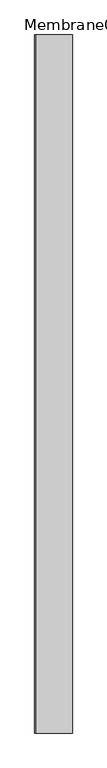
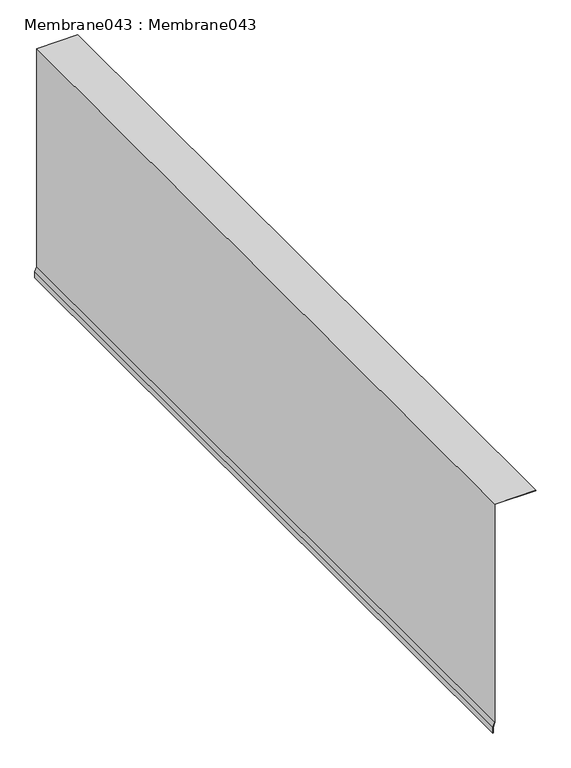
"""IFC4 building model written with IfcOpenShell, lengths in millimetres: proxy geometry, Membrane043 : Membrane043."""

from ifc_helpers import new_model, si_unit, frame, origin, place, context, project, spatial, polyline, outline, extrude, source, transform, mapped, element, save


def membrane043_membrane043_b5c9dd8e(model_context):
    return source(origin(), model_context, "Body", "SweptSolid", [
        extrude(outline(polyline([(40160.8681333, -9788.4545063), (40160.8681333, -9892.1962891), (39579.4993977, -9892.1962891), (39568.2741325, -9896.2819515), (39552.6918208, -9896.2819515), (39552.6918208, -9895.2819515), (39568.0978055, -9895.2819515), (39579.3230707, -9891.1962891), (40159.8681333, -9891.1962891), (40159.8681333, -9788.4545063), (40160.8681333, -9788.4545063)])), frame((0.0, 7982.1531721, 0.0), z_axis=(0.0, 1.0, 0.0), x_axis=(0.0, 0.0, 1.0)), (0.0, 0.0, 1.0), 2000.0),
    ])


if __name__ == "__main__":
    model = new_model("IFC4")
    model_context = context("Model", 3, world=origin())
    ifc_project = project(units=[si_unit("LENGTHUNIT", "METRE", prefix="MILLI")], contexts=[model_context])
    site = spatial("IfcSite", under=ifc_project)
    building = spatial("IfcBuilding", under=site)
    placement = place(None, origin())
    membrane043_membrane043_shape = membrane043_membrane043_b5c9dd8e(model_context)
    element("IfcBuildingElementProxy", 1, Name="Membrane043 : Membrane043", ObjectType="Membrane043 : Membrane043", at=placement, inside=building, context=model_context, shape_type="MappedRepresentation", body=[
        mapped(membrane043_membrane043_shape, transform((0.0, 0.0, 0.0), x_axis=(1.0, 0.0, 0.0), y_axis=(0.0, 1.0, 0.0), z_axis=(0.0, 0.0, 1.0))),
    ])
    save(model, "model.ifc")

# Revit data of these elements
# Type "Membrane043 : Membrane043"
#   NameOverride = "Membrane043"
# Element 1 (IfcBuildingElementProxy, "Membrane043 : Membrane043")
#   Materials on its faces: "2 LAYERS NO. 30 ASTM D226 ASPHALT SATURATED ORGANIC FELT"
# Materials
#   "2 LAYERS NO. 30 ASTM D226 ASPHALT SATURATED ORGANIC FELT": class "Unassigned", colour RGB 46 171 0, transparency 0
